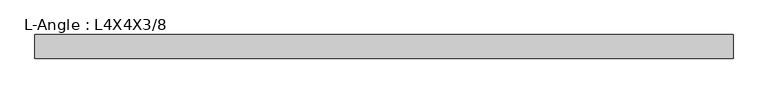
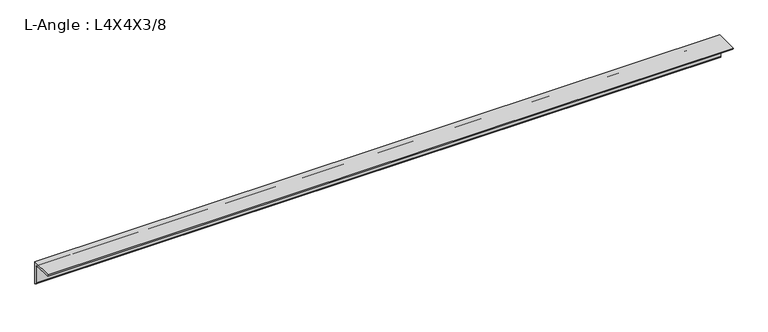
"""IFC4 building model written with IfcOpenShell, lengths in millimetres: beam geometry, L-Angle : L4X4X3/8."""

from ifc_helpers import new_model, si_unit, point, frame, frame_2d, origin, place, context, project, spatial, polyline, circle_curve, trimmed, segment, composite_curve, outline, extrude, source, transform, mapped, element, save


def l_angle_l4x4x3_8_ed507bf5(model_context):
    return source(origin(), model_context, "Body", "SweptSolid", [
        extrude(outline(composite_curve([segment(polyline([(28.702, 28.702), (28.702, -72.898)]), True, "CONTINUOUS"), segment(trimmed(circle_curve(frame_2d((28.702, -63.373)), 9.525), [point((28.702, -72.898))], [point((19.177, -63.373))], False, "CARTESIAN"), True, "CONTINUOUS"), segment(polyline([(19.177, -63.373), (19.177, 9.652)]), True, "CONTINUOUS"), segment(trimmed(circle_curve(frame_2d((9.652, 9.652)), 9.525), [point((19.177, 9.652))], [point((9.652, 19.177))], True, "CARTESIAN"), True, "CONTINUOUS"), segment(polyline([(9.652, 19.177), (-63.373, 19.177)]), True, "CONTINUOUS"), segment(trimmed(circle_curve(frame_2d((-63.373, 28.702)), 9.525), [point((-63.373, 19.177))], [point((-72.898, 28.702))], False, "CARTESIAN"), True, "CONTINUOUS"), segment(polyline([(-72.898, 28.702), (28.702, 28.702)]), True, "CONTINUOUS")], self_intersect=False)), frame((-1538.986, 0.0, 0.0), z_axis=(1.0, 0.0, 0.0), x_axis=(0.0, 1.0, 0.0)), (0.0, 0.0, 1.0), 2999.486),
    ])


if __name__ == "__main__":
    model = new_model("IFC4")
    model_context = context("Model", 3, world=origin())
    ifc_project = project(units=[si_unit("LENGTHUNIT", "METRE", prefix="MILLI")], contexts=[model_context])
    site = spatial("IfcSite", under=ifc_project)
    building = spatial("IfcBuilding", under=site)
    placement = place(None, origin())
    l_angle_l4x4x3_8_shape = l_angle_l4x4x3_8_ed507bf5(model_context)
    element("IfcBeam", 1, ObjectType="L-Angle : L4X4X3/8", at=placement, inside=building, context=model_context, shape_type="MappedRepresentation", body=[
        mapped(l_angle_l4x4x3_8_shape, transform((0.0, 0.0, 0.0), x_axis=(1.0, 0.0, 0.0), y_axis=(0.0, 1.0, 0.0), z_axis=(0.0, 0.0, 1.0))),
    ])
    save(model, "model.ifc")

# Revit data of these elements
# Type "L-Angle : L4X4X3/8"
#   Assembly Code = "B10"
#   k = 0' - 0 3/4"
#   W = 9.8
#   Length [instance default] = 5' - 0"
#   b = 0' - 4"
#   d = 0' - 4"
#   t = 0' - 0 3/8"
#   x = 0' - 1.13"
#   y = 0' - 1.13"
#   A = 0.0198611 SF
#   Structural Material [instance default] = Steel ASTM A36
# Element 1 (IfcBeam, "L-Angle : L4X4X3/8")
#   Structural Material = Steel ASTM A992
#   Materials on its faces: "Steel ASTM A992"
# Materials
#   "Steel ASTM A36": class "Metal", colour RGB 199 199 199, transparency 0, Description = "Structural steel, ASTM A36 Grade B, mill finish", Cost = 0
#   "Steel ASTM A992": class "Metal", colour RGB 199 199 199, transparency 0, Description = "Structural steel 50ksi", Cost = 0
